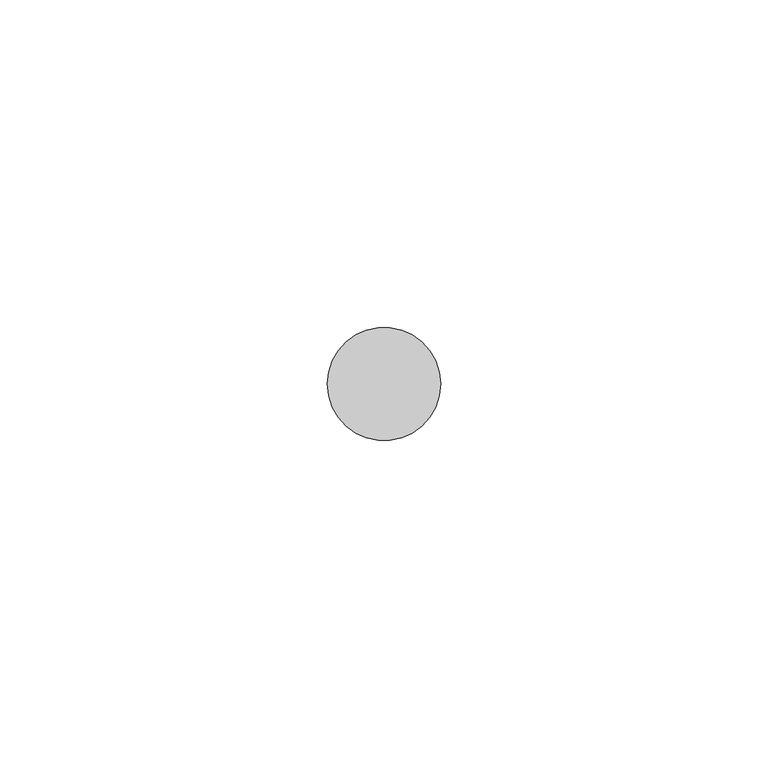
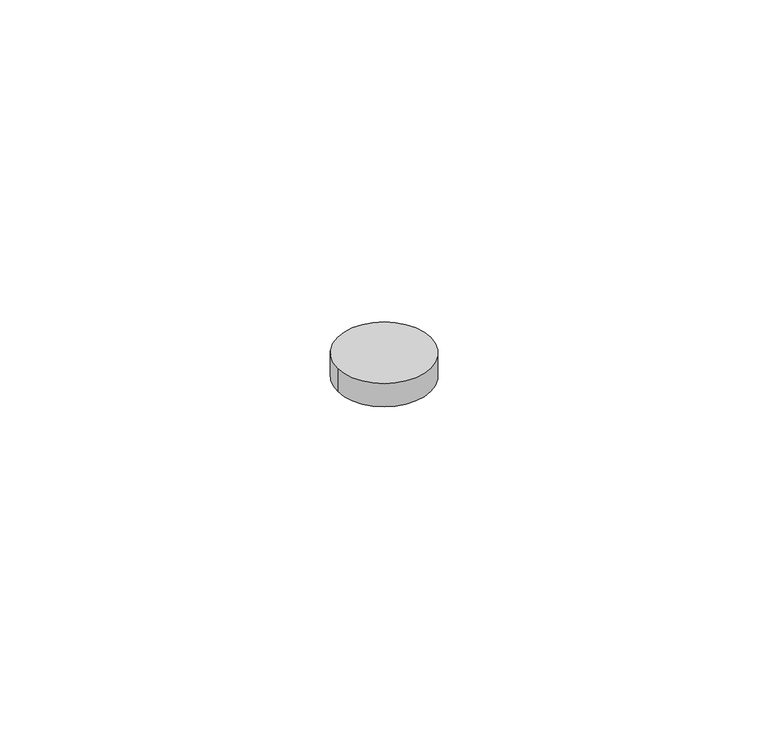
"""IFC4 building model written with IfcOpenShell, lengths in millimetres: proxy geometry, Hinge Pin Keeper2 : Hinge Pin Keeper."""

from ifc_helpers import new_model, si_unit, point, frame, frame_2d, origin, place, context, project, spatial, circle_curve, trimmed, segment, composite_curve, outline, extrude, source, transform, mapped, element, save


def generic_models_6212da49(model_context):
    return source(origin(), model_context, "Body", "SweptSolid", [
        extrude(outline(composite_curve([segment(trimmed(circle_curve(frame_2d((587319.1320739, -533984.6777841)), 8.6534625), [point((587310.4786114, -533984.6777841))], [point((587327.7855364, -533984.6777841))], False, "CARTESIAN"), True, "CONTINUOUS"), segment(trimmed(circle_curve(frame_2d((587319.1320739, -533984.6777841)), 8.6534625), [point((587327.7855364, -533984.6777841))], [point((587310.4786114, -533984.6777841))], False, "CARTESIAN"), True, "CONTINUOUS")], self_intersect=False)), frame((0.0, 0.0, 458.9859375), z_axis=(0.0, 0.0, 1.0), x_axis=(1.0, 0.0, 0.0)), (0.0, 0.0, 1.0), 4.5640625),
    ])


if __name__ == "__main__":
    model = new_model("IFC4")
    model_context = context("Model", 3, world=origin())
    ifc_project = project(units=[si_unit("LENGTHUNIT", "METRE", prefix="MILLI")], contexts=[model_context])
    site = spatial("IfcSite", under=ifc_project)
    building = spatial("IfcBuilding", under=site)
    placement = place(None, origin())
    generic_models_shape = generic_models_6212da49(model_context)
    element("IfcBuildingElementProxy", 1, Name="Hinge Pin Keeper2 : Hinge Pin Keeper", ObjectType="Hinge Pin Keeper2 : Hinge Pin Keeper", at=placement, inside=building, context=model_context, shape_type="MappedRepresentation", body=[
        mapped(generic_models_shape, transform((0.0, 0.0, 0.0), x_axis=(1.0, 0.0, 0.0), y_axis=(0.0, 1.0, 0.0), z_axis=(0.0, 0.0, 1.0))),
    ])
    save(model, "model.ifc")

# Revit data of these elements
# Element 1 (IfcBuildingElementProxy, "Hinge Pin Keeper2 : Hinge Pin Keeper")
#   Materials on its faces: "6\"X6\" WELD-ON STL BUTT HINGE"
# Materials
#   "6\"X6\" WELD-ON STL BUTT HINGE": class "Metal", colour RGB 189 187 185, transparency 0, Description = "Carbon steel", Cost = 0
